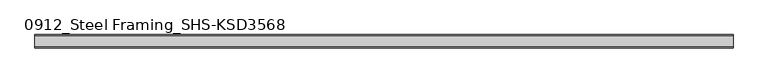
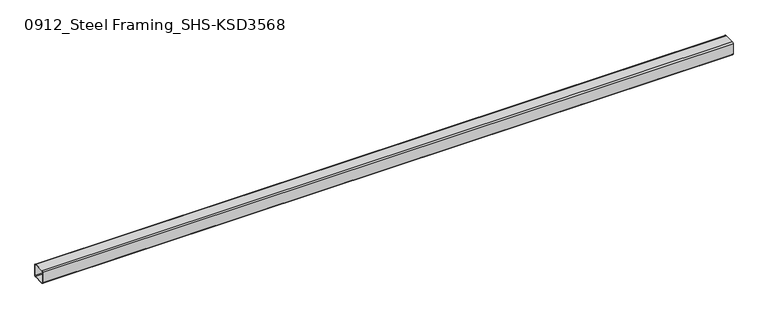
"""IFC4 building model written with IfcOpenShell, lengths in millimetres: beam geometry, 0912_Steel Framing_SHS-KSD3568 : H_SB_ASB_SHS-150x150x6."""

from ifc_helpers import new_model, si_unit, point, frame, frame_2d, origin, place, context, project, spatial, polyline, circle_curve, trimmed, segment, composite_curve, outline, extrude, source, transform, mapped, element, save


def beam_0912_steel_framing_shs_ksd3568_486cc722(model_context):
    return source(origin(), model_context, "Body", "SweptSolid", [
        extrude(outline(composite_curve([segment(polyline([(75.0, 63.0), (75.0, -63.0)]), True, "CONTINUOUS"), segment(trimmed(circle_curve(frame_2d((63.0, -63.0)), 12.0), [point((75.0, -63.0))], [point((63.0, -75.0))], False, "CARTESIAN"), True, "CONTINUOUS"), segment(polyline([(63.0, -75.0), (-63.0, -75.0)]), True, "CONTINUOUS"), segment(trimmed(circle_curve(frame_2d((-63.0, -63.0)), 12.0), [point((-63.0, -75.0))], [point((-75.0, -63.0))], False, "CARTESIAN"), True, "CONTINUOUS"), segment(polyline([(-75.0, -63.0), (-75.0, 63.0)]), True, "CONTINUOUS"), segment(trimmed(circle_curve(frame_2d((-63.0, 63.0)), 12.0), [point((-75.0, 63.0))], [point((-63.0, 75.0))], False, "CARTESIAN"), True, "CONTINUOUS"), segment(polyline([(-63.0, 75.0), (63.0, 75.0)]), True, "CONTINUOUS"), segment(trimmed(circle_curve(frame_2d((63.0, 63.0)), 12.0), [point((63.0, 75.0))], [point((75.0, 63.0))], False, "CARTESIAN"), True, "CONTINUOUS")], self_intersect=False), holes=[composite_curve([segment(trimmed(circle_curve(frame_2d((-63.0, 63.0)), 6.0), [point((-63.0, 69.0))], [point((-69.0, 63.0))], True, "CARTESIAN"), True, "CONTINUOUS"), segment(polyline([(-69.0, 63.0), (-69.0, -63.0)]), True, "CONTINUOUS"), segment(trimmed(circle_curve(frame_2d((-63.0, -63.0)), 6.0), [point((-69.0, -63.0))], [point((-63.0, -69.0))], True, "CARTESIAN"), True, "CONTINUOUS"), segment(polyline([(-63.0, -69.0), (63.0, -69.0)]), True, "CONTINUOUS"), segment(trimmed(circle_curve(frame_2d((63.0, -63.0)), 6.0), [point((63.0, -69.0))], [point((69.0, -63.0))], True, "CARTESIAN"), True, "CONTINUOUS"), segment(polyline([(69.0, -63.0), (69.0, 63.0)]), True, "CONTINUOUS"), segment(trimmed(circle_curve(frame_2d((63.0, 63.0)), 6.0), [point((69.0, 63.0))], [point((63.0, 69.0))], True, "CARTESIAN"), True, "CONTINUOUS"), segment(polyline([(63.0, 69.0), (-63.0, 69.0)]), True, "CONTINUOUS")], self_intersect=False)]), frame((-3897.5, 0.0, 0.0), z_axis=(1.0, 0.0, 0.0), x_axis=(0.0, 1.0, 0.0)), (0.0, 0.0, 1.0), 7795.0),
    ])


if __name__ == "__main__":
    model = new_model("IFC4")
    model_context = context("Model", 3, world=origin())
    ifc_project = project(units=[si_unit("LENGTHUNIT", "METRE", prefix="MILLI")], contexts=[model_context])
    site = spatial("IfcSite", under=ifc_project)
    building = spatial("IfcBuilding", under=site)
    placement = place(None, origin())
    beam_0912_steel_framing_shs_ksd3568_shape = beam_0912_steel_framing_shs_ksd3568_486cc722(model_context)
    element("IfcBeam", 1, ObjectType="0912_Steel Framing_SHS-KSD3568 : H_SB_ASB_SHS-150x150x6", at=placement, inside=building, context=model_context, shape_type="MappedRepresentation", body=[
        mapped(beam_0912_steel_framing_shs_ksd3568_shape, transform((0.0, 0.0, 0.0), x_axis=(1.0, 0.0, 0.0), y_axis=(0.0, 1.0, 0.0), z_axis=(0.0, 0.0, 1.0))),
    ])
    save(model, "model.ifc")

# Revit data of these elements
# Type "0912_Steel Framing_SHS-KSD3568 : H_SB_ASB_SHS-150x150x6"
#   H_WM Code_1 = "S01AA002-00001 | Main Steel Structure Fabrication Work | Shelter/Building | Medium Steel - Standard (90KG/M>Weight≥30KG/M) | Material: (   )"
#   H_WM Code_2 = "S03AA028-00001 | Main Steel Structure Erection Work | Shelter/Building | Medium Steel (90KG/M>Weight≥30KG/M) | Material: (   )"
#   H_WM Code_3 = "S01AA010-00001 | Main Steel Structure Fabrication Work | Shelter/Building | Steel Painting/Coating | for Non-Fireproofed Steel Surface, Surface Preparation, Primer, Second & Final Coat | Material: (   )"
#   H_Q'ty Cal Type Tag = "SB-Q2"
#   Perimeter = 0.60 m²/m
#   Nominal Weight = 26.40 kgf/m
#   Length [instance default] = 1.0000 m
#   b = 0.1500 m
#   h = 0.1500 m
#   tr = 0.0120 m
#   t = 0.0060 m
#   A = 28.36 m²
#   Structural Material [instance default] = Steel, 45-345
# Element 1 (IfcBeam, "0912_Steel Framing_SHS-KSD3568 : H_SB_ASB_SHS-150x150x6")
#   Structural Material = none
# Materials
#   "Steel, 45-345": class "Metal", colour RGB 189 187 185, transparency 0, Description = "Steel 345 MPa", Cost = 0
